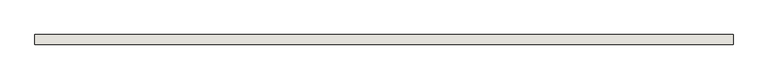
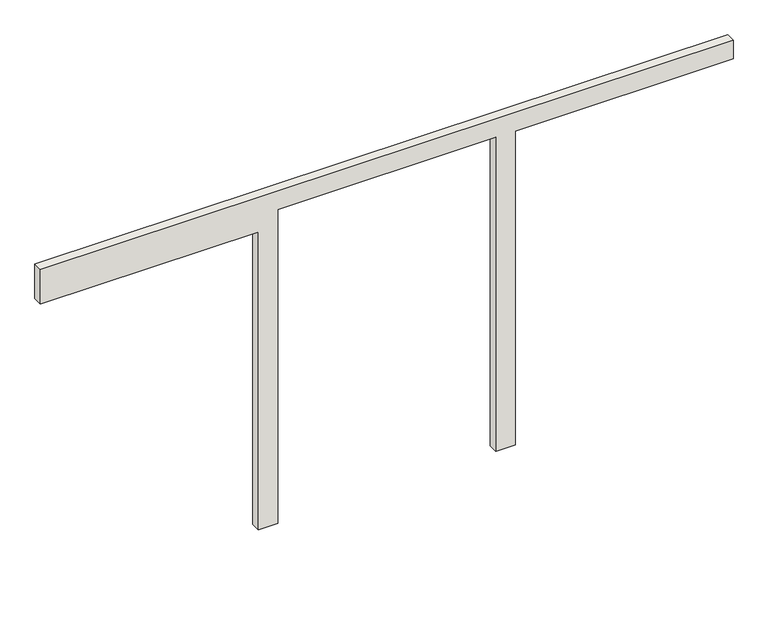
"""IFC4 building model written with IfcOpenShell, lengths in millimetres: wall geometry, 0_3d."""

from ifc_helpers import new_model, si_unit, frame, origin, place, context, project, spatial, polyline, outline, extrude, source, transform, mapped, element, save


def wall_c80d32e2(model_context):
    return source(origin(), model_context, "Body", "SweptSolid", [
        extrude(outline(polyline([(2580.0, 0.0), (2580.0, 1783.4), (0.0, 1783.4), (0.0, 1943.4), (2720.0, 1943.4), (2720.0, 3726.7), (0.0, 3726.7), (0.0, 3886.7), (2720.0, 3886.7), (2720.0, 5670.0), (2880.0, 5670.0), (2880.0, 0.0), (2580.0, 0.0)])), frame((0.0, 0.0, 0.0), z_axis=(0.0, 1.0, 0.0), x_axis=(0.0, 0.0, 1.0)), (0.0, 0.0, 1.0), 78.0),
    ])


if __name__ == "__main__":
    model = new_model("IFC4")
    model_context = context("Model", 3, world=origin())
    ifc_project = project(units=[si_unit("LENGTHUNIT", "METRE", prefix="MILLI")], contexts=[model_context])
    site = spatial("IfcSite", under=ifc_project)
    building = spatial("IfcBuilding", under=site)
    placement = place(None, origin())
    wall_shape = wall_c80d32e2(model_context)
    element("IfcWall", 1, ObjectType="0_3d", at=placement, inside=building, context=model_context, shape_type="MappedRepresentation", body=[
        mapped(wall_shape, transform((0.0, 0.0, 0.0), x_axis=(1.0, 0.0, 0.0), y_axis=(0.0, 1.0, 0.0), z_axis=(0.0, 0.0, 1.0))),
    ])
    save(model, "model.ifc")

# Revit data of these elements
# Element 1 (IfcWall, "0_3d")
#   Materials on its faces: "glas"
# Materials
#   "glas": class "Unassigned", colour RGB 250 253 254, transparency 0.95
